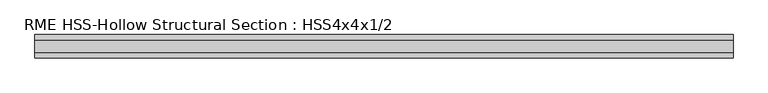
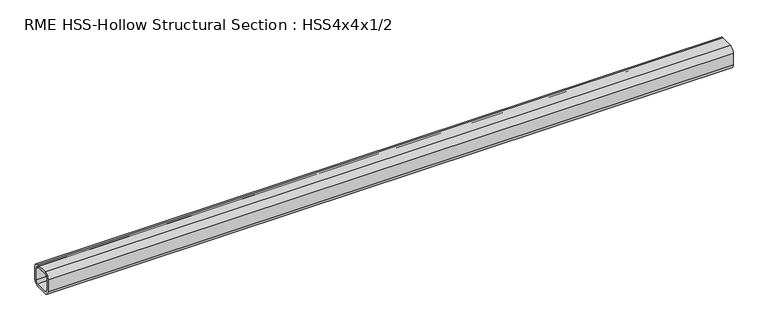
"""IFC4 building model written with IfcOpenShell, lengths in millimetres: member geometry, RME HSS-Hollow Structural Section : HSS4x4x1/2."""

from ifc_helpers import new_model, si_unit, point, frame, frame_2d, origin, place, context, project, spatial, polyline, circle_curve, trimmed, segment, composite_curve, outline, extrude, source, transform, mapped, element, save


def rme_hss_hollow_structural_section_hss4x4x1_2_754ec3d7(model_context):
    return source(origin(), model_context, "Body", "SweptSolid", [
        extrude(outline(composite_curve([segment(polyline([(50.8, 27.178), (50.8, -27.178)]), True, "CONTINUOUS"), segment(trimmed(circle_curve(frame_2d((27.178, -27.178)), 23.622), [point((50.8, -27.178))], [point((27.178, -50.8))], False, "CARTESIAN"), True, "CONTINUOUS"), segment(polyline([(27.178, -50.8), (-27.178, -50.8)]), True, "CONTINUOUS"), segment(trimmed(circle_curve(frame_2d((-27.178, -27.178)), 23.622), [point((-27.178, -50.8))], [point((-50.8, -27.178))], False, "CARTESIAN"), True, "CONTINUOUS"), segment(polyline([(-50.8, -27.178), (-50.8, 27.178)]), True, "CONTINUOUS"), segment(trimmed(circle_curve(frame_2d((-27.178, 27.178)), 23.622), [point((-50.8, 27.178))], [point((-27.178, 50.8))], False, "CARTESIAN"), True, "CONTINUOUS"), segment(polyline([(-27.178, 50.8), (27.178, 50.8)]), True, "CONTINUOUS"), segment(trimmed(circle_curve(frame_2d((27.178, 27.178)), 23.622), [point((27.178, 50.8))], [point((50.8, 27.178))], False, "CARTESIAN"), True, "CONTINUOUS")], self_intersect=False), holes=[composite_curve([segment(trimmed(circle_curve(frame_2d((-27.178, 27.178)), 11.811), [point((-27.178, 38.989))], [point((-38.989, 27.178))], True, "CARTESIAN"), True, "CONTINUOUS"), segment(polyline([(-38.989, 27.178), (-38.989, -27.178)]), True, "CONTINUOUS"), segment(trimmed(circle_curve(frame_2d((-27.178, -27.178)), 11.811), [point((-38.989, -27.178))], [point((-27.178, -38.989))], True, "CARTESIAN"), True, "CONTINUOUS"), segment(polyline([(-27.178, -38.989), (27.178, -38.989)]), True, "CONTINUOUS"), segment(trimmed(circle_curve(frame_2d((27.178, -27.178)), 11.811), [point((27.178, -38.989))], [point((38.989, -27.178))], True, "CARTESIAN"), True, "CONTINUOUS"), segment(polyline([(38.989, -27.178), (38.989, 27.178)]), True, "CONTINUOUS"), segment(trimmed(circle_curve(frame_2d((27.178, 27.178)), 11.811), [point((38.989, 27.178))], [point((27.178, 38.989))], True, "CARTESIAN"), True, "CONTINUOUS"), segment(polyline([(27.178, 38.989), (-27.178, 38.989)]), True, "CONTINUOUS")], self_intersect=False)]), frame((-1666.5527521, 0.0, 0.0), z_axis=(1.0, 0.0, 0.0), x_axis=(0.0, 1.0, 0.0)), (0.0, 0.0, 1.0), 3032.9220228),
    ])


if __name__ == "__main__":
    model = new_model("IFC4")
    model_context = context("Model", 3, world=origin())
    ifc_project = project(units=[si_unit("LENGTHUNIT", "METRE", prefix="MILLI")], contexts=[model_context])
    site = spatial("IfcSite", under=ifc_project)
    building = spatial("IfcBuilding", under=site)
    placement = place(None, origin())
    rme_hss_hollow_structural_section_hss4x4x1_2_shape = rme_hss_hollow_structural_section_hss4x4x1_2_754ec3d7(model_context)
    element("IfcMember", 1, ObjectType="RME HSS-Hollow Structural Section : HSS4x4x1/2", at=placement, inside=building, context=model_context, shape_type="MappedRepresentation", body=[
        mapped(rme_hss_hollow_structural_section_hss4x4x1_2_shape, transform((0.0, 0.0, 0.0), x_axis=(1.0, 0.0, 0.0), y_axis=(0.0, 1.0, 0.0), z_axis=(0.0, 0.0, 1.0))),
    ])
    save(model, "model.ifc")

# Revit data of these elements
# Type "RME HSS-Hollow Structural Section : HSS4x4x1/2"
#   Nominal Size = "HSS6x4"
#   Assembly Code = "B10"
#   Shape = "Square"
#   W = 21.5
#   Start Extension Calculation [instance default] = 10' - 0"
#   Start Extension [instance default] = -0' - 0 1/2"
#   End Extension Calculation [instance default] = 10' - 0"
#   End Extension [instance default] = -0' - 0 1/2"
#   Ht = 0' - 4"
#   Length [instance default] = 5' - 0"
#   b = 0' - 4"
#   kr = 0' - 0.93"
#   t = 0' - 0.465"
#   A = 0.0418056 SF
#   Structural Material [instance default] = Metal - Steel - ASTM A500 - Grade B - Rectangular and Square
# Element 1 (IfcMember, "RME HSS-Hollow Structural Section : HSS4x4x1/2")
#   End Extension Calculation = 9' - 7.3328"
#   End Extension = -0' - 5.1672"
#   Structural Material = Metal - Steel - ASTM A992
#   Materials on its faces: "Metal - Steel - ASTM A992"
# Materials
#   "Metal - Steel - ASTM A500 - Grade B - Rectangular and Square": class "Metal", colour RGB 255 128 0, transparency 0
#   "Metal - Steel - ASTM A992": class "Metal", colour RGB 255 128 0, transparency 0
